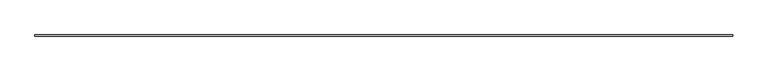
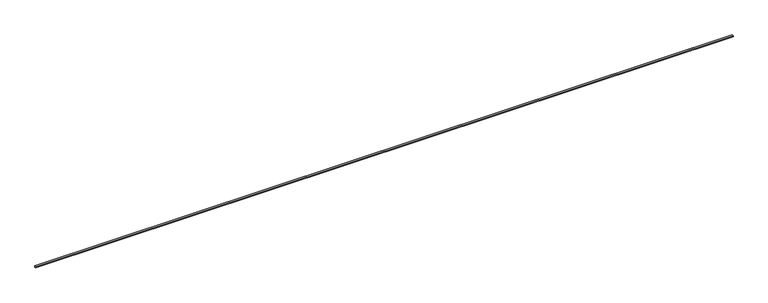
"""IFC4 building model written with IfcOpenShell, lengths in millimetres: proxy geometry, Joint009 33709 : Joint009 33709."""

from ifc_helpers import new_model, si_unit, point, frame, frame_2d, origin, place, context, project, spatial, polyline, circle_curve, trimmed, segment, composite_curve, outline, extrude, source, transform, mapped, element, save


def generic_models_4a87faaf(model_context):
    return source(origin(), model_context, "Body", "SweptSolid", [
        extrude(outline(composite_curve([segment(polyline([(-4376.7836914, 42587.1101563), (-4376.7836914, 42583.1921875)]), True, "CONTINUOUS"), segment(trimmed(circle_curve(frame_2d((-4378.3820234, 42578.0203125)), 5.4132205), [point((-4376.7836914, 42583.1921875))], [point((-4379.9803555, 42583.1921875))], True, "CARTESIAN"), True, "CONTINUOUS"), segment(polyline([(-4379.9803555, 42583.1921875), (-4379.9803555, 42587.1101563)]), True, "CONTINUOUS"), segment(trimmed(circle_curve(frame_2d((-4378.3820234, 42581.9382813)), 5.4132205), [point((-4379.9803555, 42587.1101563))], [point((-4376.7836914, 42587.1101563))], False, "CARTESIAN"), True, "CONTINUOUS")], self_intersect=False)), frame((12383.0178845, 0.0, 0.0), z_axis=(1.0, 0.0, 0.0), x_axis=(0.0, 1.0, 0.0)), (0.0, 0.0, 1.0), 2000.0),
    ])


if __name__ == "__main__":
    model = new_model("IFC4")
    model_context = context("Model", 3, world=origin())
    ifc_project = project(units=[si_unit("LENGTHUNIT", "METRE", prefix="MILLI")], contexts=[model_context])
    site = spatial("IfcSite", under=ifc_project)
    building = spatial("IfcBuilding", under=site)
    placement = place(None, origin())
    generic_models_shape = generic_models_4a87faaf(model_context)
    element("IfcBuildingElementProxy", 1, Name="Joint009 33709 : Joint009 33709", ObjectType="Joint009 33709 : Joint009 33709", at=placement, inside=building, context=model_context, shape_type="MappedRepresentation", body=[
        mapped(generic_models_shape, transform((0.0, 0.0, 0.0), x_axis=(1.0, 0.0, 0.0), y_axis=(0.0, 1.0, 0.0), z_axis=(0.0, 0.0, 1.0))),
    ])
    save(model, "model.ifc")

# Revit data of these elements
# Type "Joint009 33709 : Joint009 33709"
#   NameOverride = "Joint009"
# Element 1 (IfcBuildingElementProxy, "Joint009 33709 : Joint009 33709")
#   Materials on its faces: "SEALANT JOINT"
# Materials
#   "SEALANT JOINT": class "Unassigned", colour RGB 142 225 148, transparency 0
